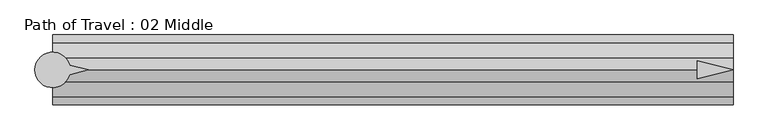
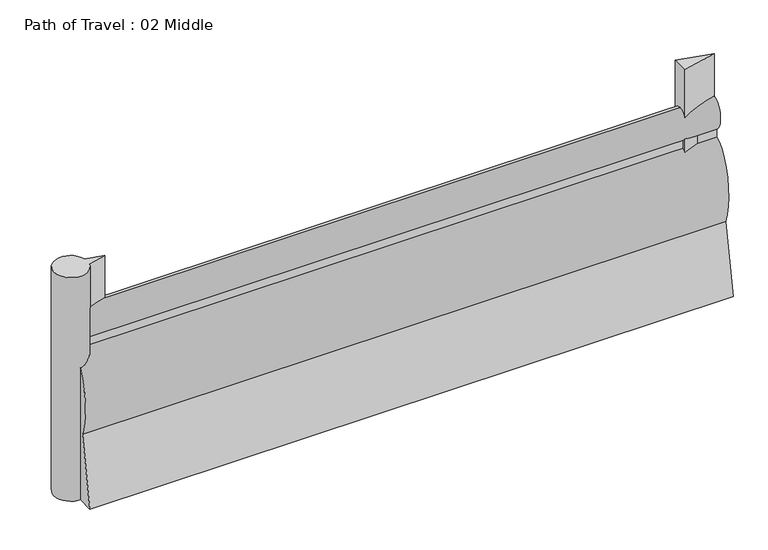
"""IFC4 building model written with IfcOpenShell, lengths in millimetres: proxy geometry, Path of Travel : 02 Middle."""

from ifc_helpers import new_model, si_unit, point, frame, frame_2d, origin, origin_with_axes, place, context, project, spatial, polyline, circle_curve, ellipse_curve, trimmed, segment, composite_curve, outline, extrude, source, transform, mapped, element, save
from ifc_brep_helpers import plane_surface, extruded_surface, advanced_brep


def path_of_travel_02_middle_495fe6d1(model_context):
    return source(origin(), model_context, "Body", "SolidModel", [
        advanced_brep(
        [(227.5554837, 0.0, 1727.2), (227.5554837, 42.9018657, 1436.6534209), (227.5554837, 42.9018657, 1363.4763406), (227.5554837, 184.1186263, 643.4144547), (227.5554837, 297.5699544, 0.0), (227.5554837, 145.6574193, 0.0), (227.5554837, 0.0, 584.2), (227.5554837, -145.6574193, 0.0), (227.5554837, -297.5699544, 0.0), (227.5554837, -184.1186263, 643.4144547), (227.5554837, -42.9018657, 1363.4763406), (227.5554837, -42.9018657, 1436.6534209), (6018.7554837, 0.0, 1727.2), (6018.7554837, -42.9018657, 1436.6534209), (6018.7554837, -42.9018657, 1363.4763406), (6018.7554837, -184.1186263, 643.4144547), (6018.7554837, -297.5699544, 0.0), (6018.7554837, -145.6574193, 0.0), (6018.7554837, 0.0, 584.2), (6018.7554837, 145.6574193, 0.0), (6018.7554837, 297.5699544, 0.0), (6018.7554837, 184.1186263, 643.4144547), (6018.7554837, 42.9018657, 1363.4763406), (6018.7554837, 42.9018657, 1436.6534209)],
        [
            (0, 1, ellipse_curve(frame((227.5554837, 0.0, 1574.8), z_axis=(-1.0, 0.0, 0.0), x_axis=(0.0, 0.0, 1.0)), 152.4, 101.6)),
            (1, 2),
            (2, 3, ellipse_curve(frame((227.5554837, 0.0, 914.4), z_axis=(-1.0, 0.0, 0.0), x_axis=(0.0, 0.0, -1.0)), 457.2, 228.6)),
            (3, 4),
            (4, 5),
            (5, 6),
            (6, 7),
            (7, 8),
            (8, 9),
            (9, 10, ellipse_curve(frame((227.5554837, 0.0, 914.4), z_axis=(-1.0, 0.0, 0.0), x_axis=(0.0, 0.0, -1.0)), 457.2, 228.6)),
            (10, 11),
            (11, 0, ellipse_curve(frame((227.5554837, 0.0, 1574.8), z_axis=(-1.0, 0.0, 0.0), x_axis=(0.0, 0.0, 1.0)), 152.4, 101.6)),
            (12, 13, ellipse_curve(frame((6018.7554837, 0.0, 1574.8), z_axis=(1.0, 0.0, 0.0), x_axis=(0.0, 0.0, 1.0)), 152.4, 101.6)),
            (13, 14),
            (14, 15, ellipse_curve(frame((6018.7554837, 0.0, 914.4), z_axis=(1.0, 0.0, 0.0), x_axis=(0.0, 0.0, -1.0)), 457.2, 228.6)),
            (15, 16),
            (16, 17),
            (17, 18),
            (18, 19),
            (19, 20),
            (20, 21),
            (21, 22, ellipse_curve(frame((6018.7554837, 0.0, 914.4), z_axis=(1.0, 0.0, 0.0), x_axis=(0.0, 0.0, -1.0)), 457.2, 228.6)),
            (22, 23),
            (23, 12, ellipse_curve(frame((6018.7554837, 0.0, 1574.8), z_axis=(1.0, 0.0, 0.0), x_axis=(0.0, 0.0, 1.0)), 152.4, 101.6)),
            (0, 12),
            (23, 1),
            (22, 2),
            (21, 3),
            (20, 4),
            (19, 5),
            (18, 6),
            (17, 7),
            (16, 8),
            (15, 9),
            (14, 10),
            (13, 11),
        ],
        [
            plane_surface(frame((227.5554837, 0.0, 0.0), z_axis=(-1.0, 0.0, 0.0), x_axis=(0.0, 0.0, 1.0))),
            plane_surface(frame((6018.7554837, 0.0, 0.0), z_axis=(1.0, 0.0, 0.0), x_axis=(0.0, 0.0, 1.0))),
            extruded_surface(trimmed(ellipse_curve(frame((6018.7554837, 0.0, 1574.8), z_axis=(-1.0, 0.0, 0.0), x_axis=(0.0, 0.0, 1.0)), 152.4, 101.6), [point((6018.7554837, 0.0, 1727.2))], [point((6018.7554837, 42.9018657, 1436.6534209))], True, "CARTESIAN"), (-5791.2, 0.0, 0.0), 5791.2),
            plane_surface(frame((227.5554837, 42.9018657, 1436.6534209), z_axis=(0.0, 1.0, 0.0), x_axis=(1.0, 0.0, 0.0))),
            extruded_surface(trimmed(ellipse_curve(frame((6018.7554837, 0.0, 914.4), z_axis=(-1.0, 0.0, 0.0), x_axis=(0.0, 0.0, -1.0)), 457.2, 228.6), [point((6018.7554837, 42.9018657, 1363.4763406))], [point((6018.7554837, 184.1186263, 643.4144547))], True, "CARTESIAN"), (-5791.2, 0.0, 0.0), 5791.2),
            plane_surface(frame((227.5554837, 184.1186263, 643.4144547), z_axis=(0.0, 0.9848077530122078, 0.1736481776669322), x_axis=(1.0, 0.0, 0.0))),
            plane_surface(frame((227.5554837, 297.5699544, 0.0), z_axis=(0.0, 0.0, -1.0), x_axis=(1.0, 0.0, 0.0))),
            plane_surface(frame((227.5554837, 145.6574193, 0.0), z_axis=(0.0, -0.9702957262760199, -0.2419218955995739), x_axis=(1.0, 0.0, 0.0))),
            plane_surface(frame((227.5554837, 0.0, 584.2), z_axis=(0.0, 0.9702957262759961, -0.24192189559966923), x_axis=(1.0, 0.0, 0.0))),
            plane_surface(frame((227.5554837, -145.6574193, 0.0), z_axis=(0.0, 0.0, -1.0), x_axis=(1.0, 0.0, 0.0))),
            plane_surface(frame((227.5554837, -297.5699544, 0.0), z_axis=(0.0, -0.984807753012208, 0.17364817766693066), x_axis=(1.0, 0.0, 0.0))),
            extruded_surface(trimmed(ellipse_curve(frame((6018.7554837, 0.0, 914.4), z_axis=(-1.0, 0.0, 0.0), x_axis=(0.0, 0.0, -1.0)), 457.2, 228.6), [point((6018.7554837, -184.1186263, 643.4144547))], [point((6018.7554837, -42.9018657, 1363.4763406))], True, "CARTESIAN"), (-5791.2, 0.0, 0.0), 5791.2),
            plane_surface(frame((227.5554837, -42.9018657, 1363.4763406), z_axis=(0.0, -1.0, 0.0), x_axis=(1.0, 0.0, 0.0))),
            extruded_surface(trimmed(ellipse_curve(frame((6018.7554837, 0.0, 1574.8), z_axis=(-1.0, 0.0, 0.0), x_axis=(0.0, 0.0, 1.0)), 152.4, 101.6), [point((6018.7554837, -42.9018657, 1436.6534209))], [point((6018.7554837, 0.0, 1727.2))], True, "CARTESIAN"), (-5791.2, 0.0, 0.0), 5791.2),
        ],
        [
            (0, [[1, 2, 3, 4, 5, 6, 7, 8, 9, 10, 11, 12]]),
            (1, [[13, 14, 15, 16, 17, 18, 19, 20, 21, 22, 23, 24]]),
            (2, [[-1, 25, -24, 26]]),
            (3, [[-2, -26, -23, 27]]),
            (4, [[-3, -27, -22, 28]]),
            (5, [[-4, -28, -21, 29]]),
            (6, [[-5, -29, -20, 30]]),
            (7, [[-6, -30, -19, 31]]),
            (8, [[-7, -31, -18, 32]]),
            (9, [[-8, -32, -17, 33]]),
            (10, [[-9, -33, -16, 34]]),
            (11, [[-10, -34, -15, 35]]),
            (12, [[-11, -35, -14, 36]]),
            (13, [[-12, -36, -13, -25]]),
        ],
    ),
        extrude(outline(polyline([(5712.7503371, 76.2006338), (6018.7554837, 0.0), (5712.7503371, -76.2006338), (5712.7503371, 76.2006338)])), origin_with_axes(), (0.0, 0.0, 1.0), 2129.5973753),
        extrude(outline(composite_curve([segment(polyline([(372.7837828, 39.4440225), (531.182385, 0.0), (372.7837828, -39.4440225)]), True, "CONTINUOUS"), segment(trimmed(circle_curve(frame_2d((227.2200886, 0.0)), 150.8131956), [point((372.7837828, -39.4440225))], [point((372.7837828, 39.4440225))], False, "CARTESIAN"), True, "CONTINUOUS")], self_intersect=False)), origin_with_axes(), (0.0, 0.0, 1.0), 2129.5973753),
    ])


if __name__ == "__main__":
    model = new_model("IFC4")
    model_context = context("Model", 3, world=origin())
    ifc_project = project(units=[si_unit("LENGTHUNIT", "METRE", prefix="MILLI")], contexts=[model_context])
    site = spatial("IfcSite", under=ifc_project)
    building = spatial("IfcBuilding", under=site)
    placement = place(None, origin())
    path_of_travel_02_middle_shape = path_of_travel_02_middle_495fe6d1(model_context)
    element("IfcBuildingElementProxy", 1, Name="Path of Travel : 02 Middle", ObjectType="Path of Travel : 02 Middle", at=placement, inside=building, context=model_context, shape_type="MappedRepresentation", body=[
        mapped(path_of_travel_02_middle_shape, transform((0.0, 0.0, 0.0), x_axis=(1.0, 0.0, 0.0), y_axis=(0.0, 1.0, 0.0), z_axis=(0.0, 0.0, 1.0))),
    ])
    save(model, "model.ifc")

# Revit data of these elements
# Type "Path of Travel : 02 Middle"
#   Path of Egress [instance default] = 4' - 0"
#   built-in parameter 1001306 [instance default] = 4 (stored number, unit not read)
#   Dot at Start = no
#   Arrow in Middle = yes
#   Arrow at End = no
#   Egress Path = none
# Element 1 (IfcBuildingElementProxy, "Path of Travel : 02 Middle")
#   Path of Egress = 19' - 0"
#   built-in parameter 1001306 = 19 (stored number, unit not read)
